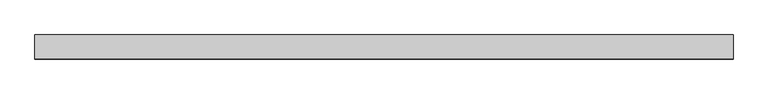
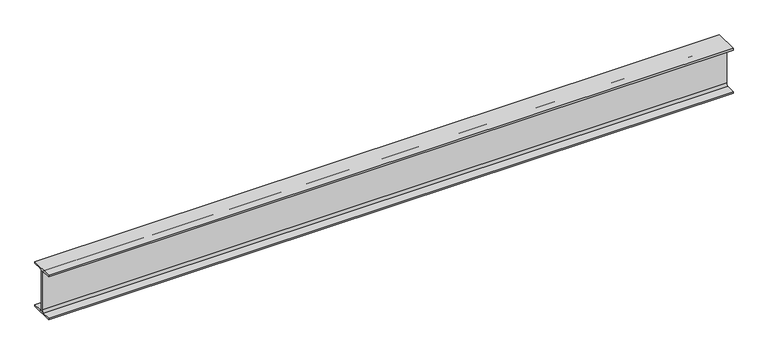
"""IFC4 building model written with IfcOpenShell, lengths in millimetres: beam geometry, 0912_Steel Framing_H-KSD3502 : H_SB_ASB_H-250x125x6x9."""

from ifc_helpers import new_model, si_unit, point, frame, frame_2d, origin, place, context, project, spatial, polyline, circle_curve, trimmed, segment, composite_curve, outline, extrude, source, transform, mapped, element, save


def beam_acfca841(model_context):
    return source(origin(), model_context, "Body", "SweptSolid", [
        extrude(outline(composite_curve([segment(polyline([(62.5, -116.0), (62.5, -125.0), (-62.5, -125.0), (-62.5, -116.0), (-15.0, -116.0)]), True, "CONTINUOUS"), segment(trimmed(circle_curve(frame_2d((-15.0, -104.0)), 12.0), [point((-15.0, -116.0))], [point((-3.0, -104.0))], True, "CARTESIAN"), True, "CONTINUOUS"), segment(polyline([(-3.0, -104.0), (-3.0, 104.0)]), True, "CONTINUOUS"), segment(trimmed(circle_curve(frame_2d((-15.0, 104.0)), 12.0), [point((-3.0, 104.0))], [point((-15.0, 116.0))], True, "CARTESIAN"), True, "CONTINUOUS"), segment(polyline([(-15.0, 116.0), (-62.5, 116.0), (-62.5, 125.0), (62.5, 125.0), (62.5, 116.0), (15.0, 116.0)]), True, "CONTINUOUS"), segment(trimmed(circle_curve(frame_2d((15.0, 104.0)), 12.0), [point((15.0, 116.0))], [point((3.0, 104.0))], True, "CARTESIAN"), True, "CONTINUOUS"), segment(polyline([(3.0, 104.0), (3.0, -104.0)]), True, "CONTINUOUS"), segment(trimmed(circle_curve(frame_2d((15.0, -104.0)), 12.0), [point((3.0, -104.0))], [point((15.0, -116.0))], True, "CARTESIAN"), True, "CONTINUOUS"), segment(polyline([(15.0, -116.0), (62.5, -116.0)]), True, "CONTINUOUS")], self_intersect=False)), frame((-1718.3833333, 0.0, 0.0), z_axis=(1.0, 0.0, 0.0), x_axis=(0.0, 1.0, 0.0)), (0.0, 0.0, 1.0), 3623.1833333),
    ])


if __name__ == "__main__":
    model = new_model("IFC4")
    model_context = context("Model", 3, world=origin())
    ifc_project = project(units=[si_unit("LENGTHUNIT", "METRE", prefix="MILLI")], contexts=[model_context])
    site = spatial("IfcSite", under=ifc_project)
    building = spatial("IfcBuilding", under=site)
    placement = place(None, origin())
    beam_shape = beam_acfca841(model_context)
    element("IfcBeam", 1, ObjectType="0912_Steel Framing_H-KSD3502 : H_SB_ASB_H-250x125x6x9", at=placement, inside=building, context=model_context, shape_type="MappedRepresentation", body=[
        mapped(beam_shape, transform((0.0, 0.0, 0.0), x_axis=(1.0, 0.0, 0.0), y_axis=(0.0, 1.0, 0.0), z_axis=(0.0, 0.0, 1.0))),
    ])
    save(model, "model.ifc")

# Revit data of these elements
# Type "0912_Steel Framing_H-KSD3502 : H_SB_ASB_H-250x125x6x9"
#   H_WM Code_1 = "S01AA003-00001 | Main Steel Structure Fabrication Work | Shelter/Building | Light Steel - Standard (30KG/M>Weight) | Material: (   )"
#   H_WM Code_2 = "S03AA029-00001 | Main Steel Structure Erection Work | Shelter/Building | Light Steel (30KG/M>Weight) | Material: (   )"
#   H_WM Code_3 = "S01AA010-00001 | Main Steel Structure Fabrication Work | Shelter/Building | Steel Painting/Coating | for Non-Fireproofed Steel Surface, Surface Preparation, Primer, Second & Final Coat | Material: (   )"
#   H_Q'ty Cal Type Tag = "SB-Q2"
#   Width = 12.5 cm
#   Web Thickness = 0.6 cm
#   Web Fillet = 1.2 cm
#   Warping Constant = 42539.8 cm⁶
#   W = 0
#   Torsional Moment of Inertia = 7.8102 cm⁴
#   Section Area = 37.66 cm²
#   Plastic Modulus weak axis = 73.1 cm³
#   Plastic Modulus strong axis = 366.0 cm³
#   Perimeter = 0.97 m²/m
#   Nominal Weight = 29.60 kgf/m
#   Moment of Inertia weak axis = 294.00 cm⁴
#   Moment of Inertia strong axis = 4050.00 cm⁴
#   Height = 25.0 cm
#   Flange Thickness = 0.9 cm
#   Elastic Modulus weak axis = 47.0 cm³
#   Elastic Modulus strong axis = 324.0 cm³
#   Centroid Vertical = 12.5 cm
#   Centroid Horizontal = 6.25 cm
#   Ix = 40500000
#   Length [instance default] = 1.5240 m
#   Zx = 366000
#   b = 0.1250 m
#   h = 0.2500 m
#   r = 0.0120 m
#   s = 0.0060 m
#   t = 0.0090 m
#   A = 0.003766 m²
#   Structural Material [instance default] = Steel, 45-345
#   Assembly Code = ""
# Element 1 (IfcBeam, "0912_Steel Framing_H-KSD3502 : H_SB_ASB_H-250x125x6x9")
#   Structural Material = none
# Materials
#   "Steel, 45-345": class "Metal", colour RGB 189 187 185, transparency 0, Description = "Steel 345 MPa", Cost = 0
